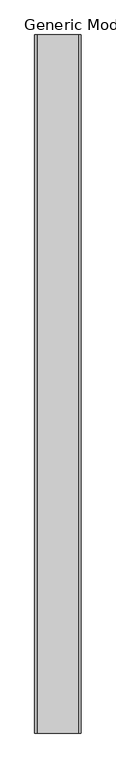
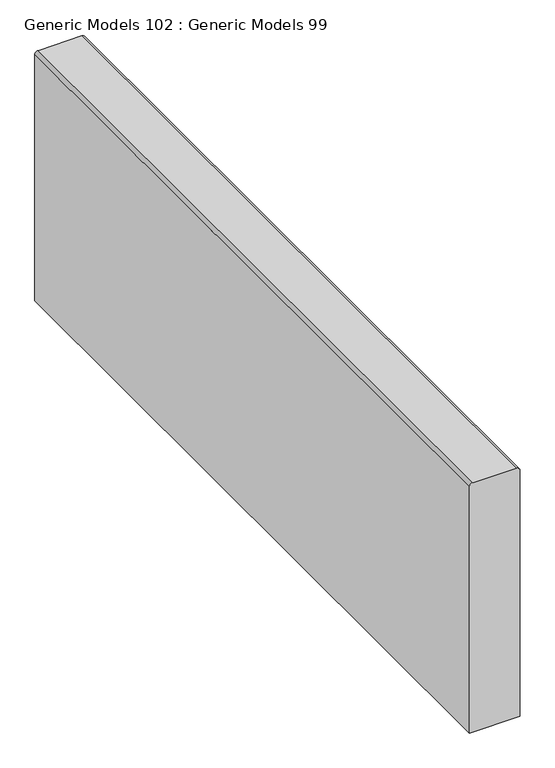
"""IFC4 building model written with IfcOpenShell, lengths in millimetres: proxy geometry, Generic Models 102 : Generic Models 99."""

from ifc_helpers import new_model, si_unit, frame, origin, place, context, project, spatial, circle_curve, source, transform, mapped, element, save
from ifc_brep_helpers import plane_surface, cylinder_surface, advanced_brep


def generic_models_102_generic_models_99_0b418c2b(model_context):
    return source(origin(), model_context, "Body", "AdvancedBrep", [
        advanced_brep(
        [(20651.0616945, 21239.2264581, 265323.3959176), (20663.7616945, 21239.2264581, 265310.6959176), (20663.7616945, 21239.2264581, 265120.1959176), (20663.7616945, 21239.2264581, 264857.0215033), (20663.7616945, 21239.2264581, 264256.5959176), (20460.5616945, 21239.2264581, 264256.5959176), (20460.5616945, 21239.2264581, 264857.0215033), (20460.5616945, 21239.2264581, 265120.1959176), (20460.5616945, 21239.2264581, 265310.6959176), (20473.2616945, 21239.2264581, 265323.3959176), (20651.0616945, 18191.2264581, 265323.3959176), (20473.2616945, 18191.2264581, 265323.3959176), (20460.5616945, 18191.2264581, 265310.6959176), (20460.5616945, 18191.2264581, 265120.1959176), (20460.5616945, 18191.2264581, 264857.0215033), (20460.5616945, 18191.2264581, 264256.5959176), (20663.7616945, 18191.2264581, 264256.5959176), (20663.7616945, 18191.2264581, 264857.0215033), (20663.7616945, 18191.2264581, 265120.1959176), (20663.7616945, 18191.2264581, 265310.6959176)],
        [
            (0, 1, circle_curve(frame((20651.0616945, 21239.2264581, 265310.6959176), z_axis=(0.0, 1.0, 0.0), x_axis=(-1.0, 0.0, 0.0)), 12.7)),
            (1, 2),
            (2, 3),
            (3, 4),
            (4, 5),
            (5, 6),
            (6, 7),
            (7, 8),
            (8, 9, circle_curve(frame((20473.2616945, 21239.2264581, 265310.6959176), z_axis=(0.0, 1.0, 0.0), x_axis=(-1.0, 0.0, 0.0)), 12.7)),
            (9, 0),
            (10, 11),
            (11, 12, circle_curve(frame((20473.2616945, 18191.2264581, 265310.6959176), z_axis=(0.0, -1.0, 0.0), x_axis=(-1.0, 0.0, 0.0)), 12.7)),
            (12, 13),
            (13, 14),
            (14, 15),
            (15, 16),
            (16, 17),
            (17, 18),
            (18, 19),
            (19, 10, circle_curve(frame((20651.0616945, 18191.2264581, 265310.6959176), z_axis=(0.0, -1.0, 0.0), x_axis=(-1.0, 0.0, 0.0)), 12.7)),
            (1, 19),
            (16, 4),
            (15, 5),
            (12, 8),
            (9, 11),
            (10, 0),
        ],
        [
            plane_surface(frame((20638.3616945, 21239.2264581, 265310.6959176), z_axis=(0.0, 1.0, 0.0), x_axis=(0.0, 0.0, 1.0))),
            plane_surface(frame((20638.3616945, 18191.2264581, 265310.6959176), z_axis=(0.0, -1.0, 0.0), x_axis=(0.0, 0.0, -1.0))),
            plane_surface(frame((20663.7616945, 21239.2264581, 265310.6959176), z_axis=(1.0, 0.0, 0.0), x_axis=(0.0, -1.0, 0.0))),
            plane_surface(frame((20663.7616945, 21239.2264581, 264256.5959176), z_axis=(0.0, 0.0, -1.0), x_axis=(0.0, -1.0, 0.0))),
            plane_surface(frame((20460.5616945, 21239.2264581, 264256.5959176), z_axis=(-1.0, 0.0, 0.0), x_axis=(0.0, -1.0, 0.0))),
            plane_surface(frame((20473.2616945, 21239.2264581, 265323.3959176), z_axis=(0.0, 0.0, 1.0), x_axis=(0.0, -1.0, 0.0))),
            cylinder_surface(frame((20651.0616945, 18191.2264581, 265310.6959176), z_axis=(0.0, 1.0, 0.0), x_axis=(-1.0, 0.0, 0.0)), 12.7),
            cylinder_surface(frame((20473.2616945, 18191.2264581, 265310.6959176), z_axis=(0.0, 1.0, 0.0), x_axis=(-1.0, 0.0, 0.0)), 12.7),
        ],
        [
            (0, [[1, 2, 3, 4, 5, 6, 7, 8, 9, 10]]),
            (1, [[11, 12, 13, 14, 15, 16, 17, 18, 19, 20]]),
            (2, [[-4, -3, -2, 21, -19, -18, -17, 22]]),
            (3, [[-5, -22, -16, 23]]),
            (4, [[-8, -7, -6, -23, -15, -14, -13, 24]]),
            (5, [[-10, 25, -11, 26]]),
            (6, [[-1, -26, -20, -21]]),
            (7, [[-9, -24, -12, -25]]),
        ],
    ),
    ])


if __name__ == "__main__":
    model = new_model("IFC4")
    model_context = context("Model", 3, world=origin())
    ifc_project = project(units=[si_unit("LENGTHUNIT", "METRE", prefix="MILLI")], contexts=[model_context])
    site = spatial("IfcSite", under=ifc_project)
    building = spatial("IfcBuilding", under=site)
    placement = place(None, origin())
    generic_models_102_generic_models_99_shape = generic_models_102_generic_models_99_0b418c2b(model_context)
    element("IfcBuildingElementProxy", 1, Name="Generic Models 102 : Generic Models 99", ObjectType="Generic Models 102 : Generic Models 99", at=placement, inside=building, context=model_context, shape_type="MappedRepresentation", body=[
        mapped(generic_models_102_generic_models_99_shape, transform((0.0, 0.0, 0.0), x_axis=(1.0, 0.0, 0.0), y_axis=(0.0, 1.0, 0.0), z_axis=(0.0, 0.0, 1.0))),
    ])
    save(model, "model.ifc")

# Revit data of these elements
# Element 1 (IfcBuildingElementProxy, "Generic Models 102 : Generic Models 99")
#   Materials on its faces: "8\" X 3'-6\" DEEP CONCRETE FENCE FOUNDATION (6\" CURB ABOVE GRADE)"
# Materials
#   "8\" X 3'-6\" DEEP CONCRETE FENCE FOUNDATION (6\" CURB ABOVE GRADE)": class "Concrete", colour RGB 192 192 192, transparency 0, Description = "Cast-in-place concrete", Cost = 0
